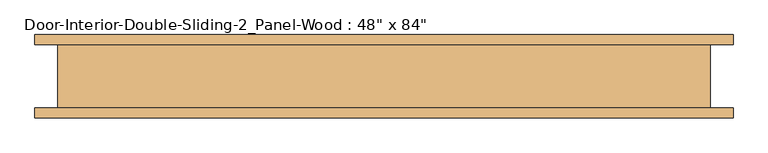
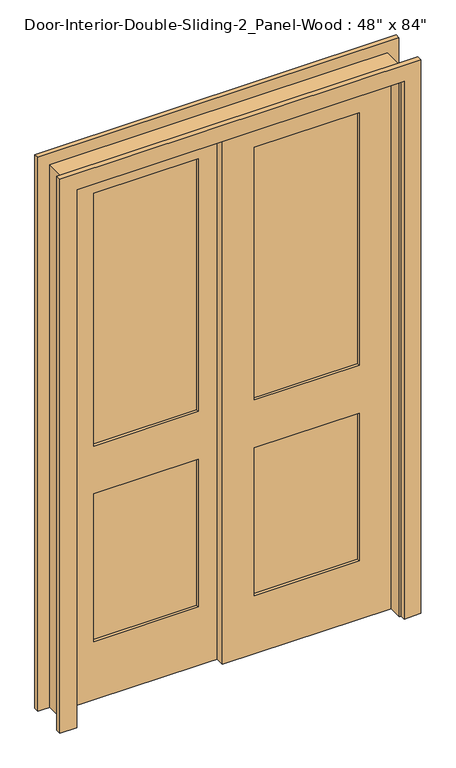
"""IFC4 building model written with IfcOpenShell, lengths in millimetres: door geometry."""

from ifc_helpers import new_model, si_unit, frame, origin, place, context, project, spatial, polyline, outline, extrude, source, transform, mapped, element, save


def door_f0c8ed54(model_context):
    return source(origin(), model_context, "Body", "SweptSolid", [
        extrude(outline(polyline([(488.95, 0.5291667), (95.25, 0.5291667), (95.25, 12.1708333), (488.95, 12.1708333), (488.95, 0.5291667)])), frame((0.0, 0.0, 1009.65), z_axis=(0.0, 0.0, 1.0), x_axis=(1.0, 0.0, 0.0)), (0.0, 0.0, 1.0), 1004.8875),
        extrude(outline(polyline([(488.95, 0.5291667), (95.25, 0.5291667), (95.25, 12.1708333), (488.95, 12.1708333), (488.95, 0.5291667)])), frame((0.0, 0.0, 231.775), z_axis=(0.0, 0.0, 1.0), x_axis=(1.0, 0.0, 0.0)), (0.0, 0.0, 1.0), 587.375),
        extrude(outline(polyline([(2133.6, -25.4), (0.0, -25.4), (0.0, 609.6), (2133.6, 609.6), (2133.6, -25.4)]), holes=[polyline([(2014.5375, 95.25), (2014.5375, 488.95), (1009.65, 488.95), (1009.65, 95.25), (2014.5375, 95.25)]), polyline([(819.15, 95.25), (819.15, 488.95), (231.775, 488.95), (231.775, 95.25), (819.15, 95.25)])]), frame((0.0, -11.1125, 0.0), z_axis=(0.0, 1.0, 0.0), x_axis=(0.0, 0.0, 1.0)), (0.0, 0.0, 1.0), 34.925),
        extrude(outline(polyline([(-95.25, 35.4541667), (-488.95, 35.4541667), (-488.95, 47.0958333), (-95.25, 47.0958333), (-95.25, 35.4541667)])), frame((0.0, 0.0, 1009.65), z_axis=(0.0, 0.0, 1.0), x_axis=(1.0, 0.0, 0.0)), (0.0, 0.0, 1.0), 1004.8875),
        extrude(outline(polyline([(-95.25, 35.4541667), (-488.95, 35.4541667), (-488.95, 47.0958333), (-95.25, 47.0958333), (-95.25, 35.4541667)])), frame((0.0, 0.0, 231.775), z_axis=(0.0, 0.0, 1.0), x_axis=(1.0, 0.0, 0.0)), (0.0, 0.0, 1.0), 587.375),
        extrude(outline(polyline([(2133.6, -609.6), (0.0, -609.6), (0.0, 25.4), (2133.6, 25.4), (2133.6, -609.6)]), holes=[polyline([(2014.5375, -488.95), (2014.5375, -95.25), (1009.65, -95.25), (1009.65, -488.95), (2014.5375, -488.95)]), polyline([(819.15, -488.95), (819.15, -95.25), (231.775, -95.25), (231.775, -488.95), (819.15, -488.95)])]), frame((0.0, 23.8125, 0.0), z_axis=(0.0, 1.0, 0.0), x_axis=(0.0, 0.0, 1.0)), (0.0, 0.0, 1.0), 34.925),
        extrude(outline(polyline([(0.0, 609.6), (0.0, 635.0), (2159.0, 635.0), (2159.0, -635.0), (0.0, -635.0), (0.0, -609.6), (2133.6, -609.6), (2133.6, 609.6), (0.0, 609.6)])), frame((0.0, -65.0875, 0.0), z_axis=(0.0, 1.0, 0.0), x_axis=(0.0, 0.0, 1.0)), (0.0, 0.0, 1.0), 123.825),
        extrude(outline(polyline([(0.0, 615.95), (0.0, 679.45), (2203.45, 679.45), (2203.45, -679.45), (0.0, -679.45), (0.0, -615.95), (2139.95, -615.95), (2139.95, 615.95), (0.0, 615.95)])), frame((0.0, -84.1375, 0.0), z_axis=(0.0, 1.0, 0.0), x_axis=(0.0, 0.0, 1.0)), (0.0, 0.0, 1.0), 19.05),
        extrude(outline(polyline([(0.0, 615.95), (0.0, 679.45), (2203.45, 679.45), (2203.45, -679.45), (0.0, -679.45), (0.0, -615.95), (2139.95, -615.95), (2139.95, 615.95), (0.0, 615.95)])), frame((0.0, 58.7375, 0.0), z_axis=(0.0, 1.0, 0.0), x_axis=(0.0, 0.0, 1.0)), (0.0, 0.0, 1.0), 19.05),
    ])


if __name__ == "__main__":
    model = new_model("IFC4")
    model_context = context("Model", 3, world=origin())
    ifc_project = project(units=[si_unit("LENGTHUNIT", "METRE", prefix="MILLI")], contexts=[model_context])
    site = spatial("IfcSite", under=ifc_project)
    building = spatial("IfcBuilding", under=site)
    placement = place(None, origin())
    door_shape = door_f0c8ed54(model_context)
    element("IfcDoor", 1, ObjectType="Door-Interior-Double-Sliding-2_Panel-Wood : 48\" x 84\"", at=placement, inside=building, context=model_context, shape_type="MappedRepresentation", body=[
        mapped(door_shape, transform((0.0, 0.0, 0.0), x_axis=(1.0, 0.0, 0.0), y_axis=(0.0, 1.0, 0.0), z_axis=(0.0, 0.0, 1.0))),
    ])
    save(model, "model.ifc")

# Revit data of these elements
# Type "Door-Interior-Double-Sliding-2_Panel-Wood : 48\" x 84\""
#   Type Mark = "21"
#   Assembly Code = "C1020300"
#   Analytic Construction = "Wooden"
#   Top Rail = 0' - 4 11/16"
#   Thickness = 0' - 1 3/8"
#   Thermal Resistance (R) = 2.5876 (h·ft²·°F)/BTU
#   Stiles = 0' - 4 3/4"
#   Rough Width = 4' - 2"
#   Rough Height = 7' - 1"
#   Lock Rail = 0' - 7 1/2"
#   Height = 7' - 0"
#   Width = 4' - 0"
#   Heat Transfer Coefficient (U) = 0.3865 BTU/(h·ft²·°F)
#   Bottom Rail = 0' - 9 1/8"
#   Trim Material = Cherry
#   Panel Material = Cherry
#   Frame Material = Cherry
#   Visual Light Transmittance = 0
#   Solar Heat Gain Coefficient = 0
#   Wall Closure = (empty or 0)
#   Function = (empty or 0)
# Element 1 (IfcDoor, "Door-Interior-Double-Sliding-2_Panel-Wood : 48\" x 84\"")
#   Materials on its faces: "Cherry"
# Materials
#   "Cherry": class "Wood", colour RGB 226 177 128, transparency 0, Description = "Prunus Serotina", Cost = 0
